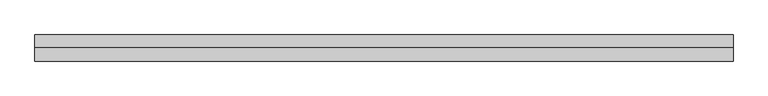
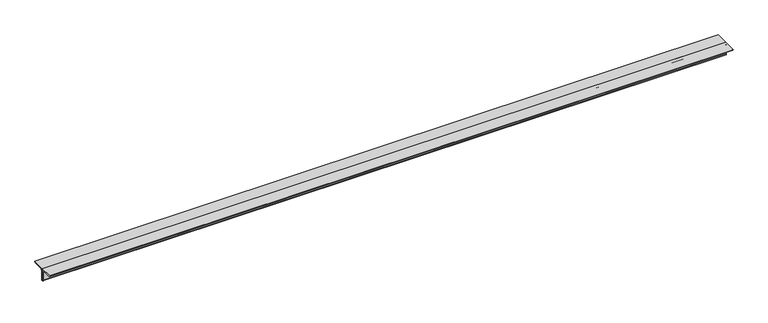
"""IFC4 building model written with IfcOpenShell, lengths in millimetres: member geometry, Steel Framing_2Ls_KS : H_SB_AR_S02_2Ls-100x100x10_VBR1."""

from ifc_helpers import new_model, si_unit, point, frame, frame_2d, origin, place, context, project, spatial, polyline, circle_curve, trimmed, segment, composite_curve, outline, extrude, source, transform, mapped, element, save


def member_17ddce70(model_context):
    return source(origin(), model_context, "Body", "SweptSolid", [
        extrude(outline(composite_curve([segment(polyline([(0.0, 28.2), (0.0, -71.8)]), True, "CONTINUOUS"), segment(trimmed(circle_curve(frame_2d((0.0, -61.8)), 10.0), [point((0.0, -71.8))], [point((-10.0, -61.8))], False, "CARTESIAN"), True, "CONTINUOUS"), segment(polyline([(-10.0, -61.8), (-10.0, 8.2)]), True, "CONTINUOUS"), segment(trimmed(circle_curve(frame_2d((-20.0, 8.2)), 10.0), [point((-10.0, 8.2))], [point((-20.0, 18.2))], True, "CARTESIAN"), True, "CONTINUOUS"), segment(polyline([(-20.0, 18.2), (-90.0, 18.2)]), True, "CONTINUOUS"), segment(trimmed(circle_curve(frame_2d((-90.0, 28.2)), 10.0), [point((-90.0, 18.2))], [point((-100.0, 28.2))], False, "CARTESIAN"), True, "CONTINUOUS"), segment(polyline([(-100.0, 28.2), (0.0, 28.2)]), True, "CONTINUOUS")], self_intersect=False)), frame((-2590.3354834, 0.0, 0.0), z_axis=(1.0, 0.0, 0.0), x_axis=(0.0, 1.0, 0.0)), (0.0, 0.0, 1.0), 5345.6471524),
        extrude(outline(composite_curve([segment(polyline([(0.0, 28.2), (100.0, 28.2)]), True, "CONTINUOUS"), segment(trimmed(circle_curve(frame_2d((90.0, 28.2)), 10.0), [point((100.0, 28.2))], [point((90.0, 18.2))], False, "CARTESIAN"), True, "CONTINUOUS"), segment(polyline([(90.0, 18.2), (20.0, 18.2)]), True, "CONTINUOUS"), segment(trimmed(circle_curve(frame_2d((20.0, 8.2)), 10.0), [point((20.0, 18.2))], [point((10.0, 8.2))], True, "CARTESIAN"), True, "CONTINUOUS"), segment(polyline([(10.0, 8.2), (10.0, -61.8)]), True, "CONTINUOUS"), segment(trimmed(circle_curve(frame_2d((0.0, -61.8)), 10.0), [point((10.0, -61.8))], [point((0.0, -71.8))], False, "CARTESIAN"), True, "CONTINUOUS"), segment(polyline([(0.0, -71.8), (0.0, 28.2)]), True, "CONTINUOUS")], self_intersect=False)), frame((-2590.3354834, 0.0, 0.0), z_axis=(1.0, 0.0, 0.0), x_axis=(0.0, 1.0, 0.0)), (0.0, 0.0, 1.0), 5345.6471524),
    ])


if __name__ == "__main__":
    model = new_model("IFC4")
    model_context = context("Model", 3, world=origin())
    ifc_project = project(units=[si_unit("LENGTHUNIT", "METRE", prefix="MILLI")], contexts=[model_context])
    site = spatial("IfcSite", under=ifc_project)
    building = spatial("IfcBuilding", under=site)
    placement = place(None, origin())
    member_shape = member_17ddce70(model_context)
    element("IfcMember", 1, ObjectType="Steel Framing_2Ls_KS : H_SB_AR_S02_2Ls-100x100x10_VBR1", at=placement, inside=building, context=model_context, shape_type="MappedRepresentation", body=[
        mapped(member_shape, transform((0.0, 0.0, 0.0), x_axis=(1.0, 0.0, 0.0), y_axis=(0.0, 1.0, 0.0), z_axis=(0.0, 0.0, 1.0))),
    ])
    save(model, "model.ifc")

# Revit data of these elements
# Type "Steel Framing_2Ls_KS : H_SB_AR_S02_2Ls-100x100x10_VBR1"
#   Type Comments = "MAIN"
#   Type Mark = "VBR1"
#   H_SectionID = "2Ls-100x100x10"
#   Assembly Code = "B10"
#   Legs = "LLBB"
#   H_Ratio for Additional Steel Plate = 0.2
#   W = 0
#   Perimeter = 0.80 m²/m
#   Nominal Weight = 29.80 kgf/m
#   Length [instance default] = 1524 mm
#   Space = 0 mm
#   b = 100 mm
#   d = 100 mm
#   t = 10 mm
#   y = 28.2 mm
#   A = 0.0038 m²
#   Structural Material [instance default] = Steel, 45-345
# Element 1 (IfcMember, "Steel Framing_2Ls_KS : H_SB_AR_S02_2Ls-100x100x10_VBR1")
#   Materials on its faces: "Steel, 45-345"
# Materials
#   "Steel, 45-345": class "Metal", colour RGB 189 187 185, transparency 0, Description = "Steel 345 MPa", Cost = 0
